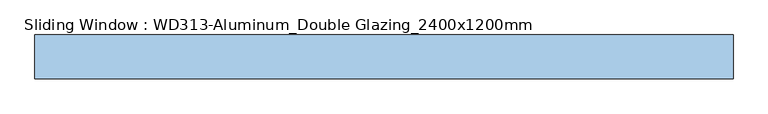
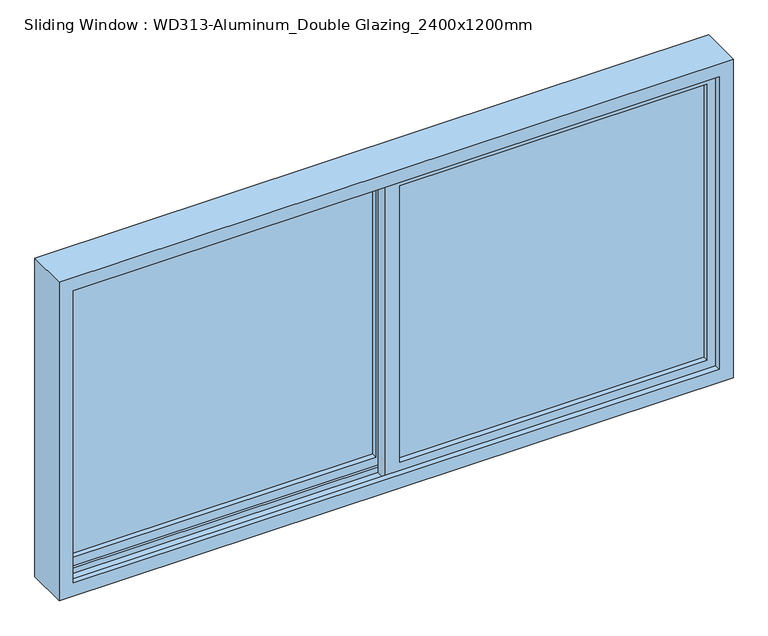
"""IFC4 building model written with IfcOpenShell, lengths in millimetres: window geometry, Sliding Window : WD313-Aluminum_Double Glazing_2400x1200mm."""

from ifc_helpers import new_model, si_unit, frame, origin, place, context, project, spatial, polyline, outline, extrude, faceted_brep, source, transform, mapped, element, save


def sliding_window_wd313_aluminum_double_glazing_2400x1200mm_8df35650(model_context):
    return source(origin(), model_context, "Body", "SolidModel", [
        extrude(outline(polyline([(1120.0, -27.5), (1120.0, -32.5), (25.0, -32.5), (25.0, -27.5), (1120.0, -27.5)])), frame((0.0, 0.0, 680.0), z_axis=(0.0, 0.0, 1.0), x_axis=(1.0, 0.0, 0.0)), (0.0, 0.0, 1.0), 1040.0),
        extrude(outline(polyline([(-25.0, 32.5), (-25.0, 27.5), (-1120.0, 27.5), (-1120.0, 32.5), (-25.0, 32.5)])), frame((0.0, 0.0, 680.0), z_axis=(0.0, 0.0, 1.0), x_axis=(1.0, 0.0, 0.0)), (0.0, 0.0, 1.0), 1040.0),
        extrude(outline(polyline([(1770.0, -1170.0), (630.0, -1170.0), (630.0, 25.0), (1770.0, 25.0), (1770.0, -1170.0)]), holes=[polyline([(680.0, -1120.0), (1720.0, -1120.0), (1720.0, -25.0), (680.0, -25.0), (680.0, -1120.0)])]), frame((0.0, 7.5, 0.0), z_axis=(0.0, 1.0, 0.0), x_axis=(0.0, 0.0, 1.0)), (0.0, 0.0, 1.0), 47.5),
        extrude(outline(polyline([(1770.0, -25.0), (630.0, -25.0), (630.0, 1170.0), (1770.0, 1170.0), (1770.0, -25.0)]), holes=[polyline([(680.0, 25.0), (1720.0, 25.0), (1720.0, 1120.0), (680.0, 1120.0), (680.0, 25.0)])]), frame((0.0, -52.5, 0.0), z_axis=(0.0, 1.0, 0.0), x_axis=(0.0, 0.0, 1.0)), (0.0, 0.0, 1.0), 45.0),
        faceted_brep([(-1200.0, -75.0, 1800.0), (-1200.0, 75.0, 1800.0), (-1200.0, 75.0, 600.0), (-1200.0, -75.0, 600.0), (1200.0, -75.0, 1800.0), (1200.0, -75.0, 600.0), (1150.0, -75.0, 650.0), (-1150.0, -75.0, 650.0), (-1150.0, -75.0, 1750.0), (1150.0, -75.0, 1750.0), (1200.0, 75.0, 600.0), (1200.0, 75.0, 1800.0), (-1150.0, 75.0, 1750.0), (-1150.0, 75.0, 650.0), (1150.0, 75.0, 650.0), (1150.0, 75.0, 1750.0), (1150.0, -55.0, 1750.0), (1150.0, -55.0, 650.0), (-1150.0, -55.0, 650.0), (-1150.0, -55.0, 630.0), (-1150.0, -5.0, 630.0), (-1150.0, -5.0, 650.0), (-1150.0, 5.0, 650.0), (-1150.0, 5.0, 1750.0), (-1150.0, -5.0, 1750.0), (-1150.0, -5.0, 1770.0), (-1150.0, -55.0, 1770.0), (-1150.0, -55.0, 1750.0), (1150.0, 5.0, 650.0), (1150.0, -5.0, 650.0), (1150.0, -5.0, 1750.0), (1150.0, 5.0, 1750.0), (1150.0, 5.0, 1770.0), (1150.0, 55.0, 1770.0), (1150.0, 55.0, 1750.0), (1150.0, 55.0, 650.0), (1150.0, 55.0, 630.0), (1150.0, 5.0, 630.0), (1170.0, -5.0, 630.0), (1170.0, -5.0, 1770.0), (-1170.0, 5.0, 1770.0), (-1170.0, 5.0, 630.0), (1170.0, -55.0, 630.0), (1170.0, -55.0, 1770.0), (-1170.0, 55.0, 630.0), (-1150.0, 55.0, 1750.0), (-1170.0, 55.0, 1770.0), (-1150.0, 55.0, 650.0)], [[[0, 1, 2, 3]], [[4, 0, 3, 5], [6, 7, 8, 9]], [[3, 2, 10, 5]], [[10, 2, 1, 11], [12, 13, 14, 15]], [[9, 16, 17, 6]], [[7, 18, 19, 20, 21, 22, 23, 24, 25, 26, 27, 8]], [[17, 18, 7, 6]], [[5, 10, 11, 4]], [[28, 22, 21, 29]], [[28, 29, 30, 31, 32, 33, 34, 15, 14, 35, 36, 37]], [[29, 21, 20, 38, 39, 25, 24, 30]], [[40, 32, 31, 23, 22, 28, 37, 41]], [[38, 42, 43, 39]], [[38, 20, 19, 42]], [[42, 19, 18, 17, 16, 27, 26, 43]], [[41, 37, 36, 44]], [[45, 34, 33, 46, 44, 36, 35, 47]], [[47, 35, 14, 13]], [[12, 45, 47, 13]], [[46, 40, 41, 44]], [[1, 0, 4, 11]], [[30, 24, 23, 31]], [[43, 26, 25, 39]], [[9, 8, 27, 16]], [[12, 15, 34, 45]], [[46, 33, 32, 40]]]),
    ])


if __name__ == "__main__":
    model = new_model("IFC4")
    model_context = context("Model", 3, world=origin())
    ifc_project = project(units=[si_unit("LENGTHUNIT", "METRE", prefix="MILLI")], contexts=[model_context])
    site = spatial("IfcSite", under=ifc_project)
    building = spatial("IfcBuilding", under=site)
    placement = place(None, origin())
    sliding_window_wd313_aluminum_double_glazing_2400x1200mm_shape = sliding_window_wd313_aluminum_double_glazing_2400x1200mm_8df35650(model_context)
    element("IfcWindow", 1, ObjectType="Sliding Window : WD313-Aluminum_Double Glazing_2400x1200mm", at=placement, inside=building, context=model_context, shape_type="MappedRepresentation", body=[
        mapped(sliding_window_wd313_aluminum_double_glazing_2400x1200mm_shape, transform((0.0, 0.0, 0.0), x_axis=(1.0, 0.0, 0.0), y_axis=(0.0, 1.0, 0.0), z_axis=(0.0, 0.0, 1.0))),
    ])
    save(model, "model.ifc")

# Revit data of these elements
# Type "Sliding Window : WD313-Aluminum_Double Glazing_2400x1200mm"
#   Type Mark = "PW"
#   Analytic Construction = "<None>"
#   창 두께 = 150 mm
#   Visual Light Transmittance = 0.9
#   Thermal Resistance (R) = 0.271106 (m²·K)/W
#   Solar Heat Gain Coefficient = 0.78
#   Height = 1200 mm
#   Heat Transfer Coefficient (U) = 3.6886 W/(m²·K)
#   기본 씰 높이 = 600 mm
#   Width = 2400 mm
#   Define Thermal Properties by = 1
#   창 패널 = AW1 창 패널
#   창 프레임 = A04AQ127-00002_Aluminum Window_None FP
#   Description = (empty or 0)
#   Construction Type Id = ""
#   Wall Closure = (empty or 0)
# Element 1 (IfcWindow, "Sliding Window : WD313-Aluminum_Double Glazing_2400x1200mm")
#   Materials on its faces: "A04AQ127-00002_Aluminum Window_None FP", "AW1 창 패널"
# Materials
#   "AW1 창 패널": class "유리", colour RGB 0 0 255, transparency 0.75
#   "A04AQ127-00002_Aluminum Window_None FP": class "금속", colour RGB 247 247 247, transparency 0, W00) Work Master Code = "A04AQ127-00002", W01) Work Master_Lv1 = "Finishing Work", W02) Work Master_Lv2 = "Door & Window Work", W03) Work Master_Spec.1 = "Aluminum Window", W04) Work Master_Spec.2 = "Fire Protective Rating: N/A", W05) Work Master_Spec.3 = "w/ Hardware & Accessories", Cost = 0
